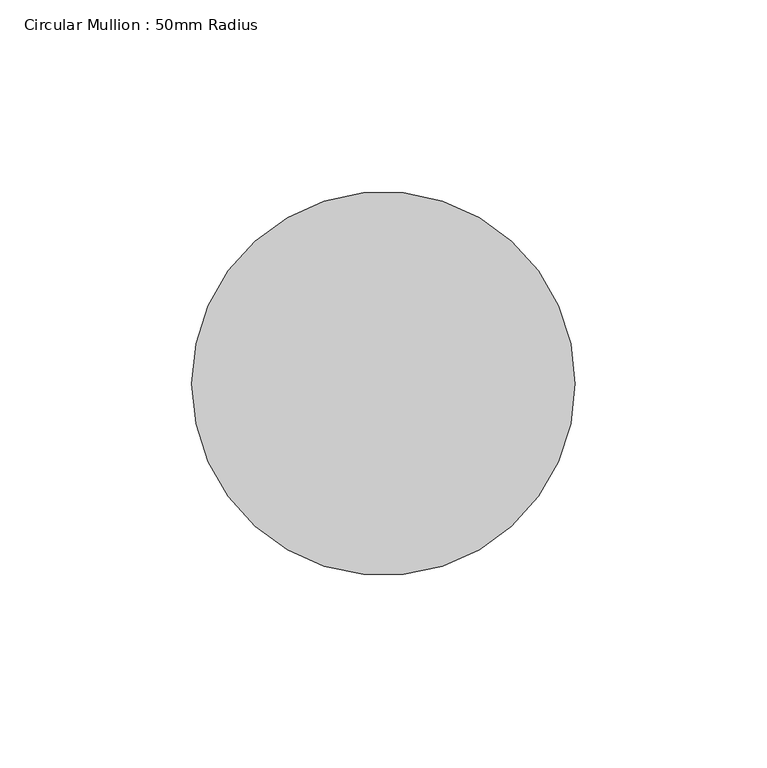
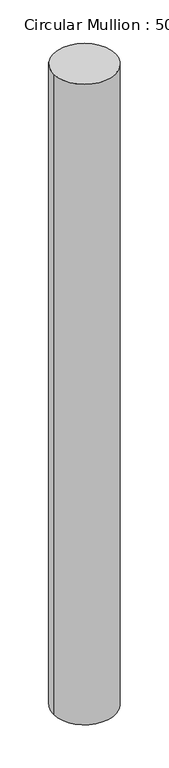
"""IFC4 building model written with IfcOpenShell, lengths in millimetres: member geometry, Circular Mullion : 50mm Radius."""

import ifcopenshell
import ifcopenshell.guid

model = None  # the IFC model being written
_history = None  # IfcOwnerHistory: only IFC2X3 demands one
_inside = {}  # id of a spatial element -> (the spatial element, [elements in it])
_under = {}  # id of a project, library or spatial element -> (it, [spatial elements below it])
_declared = {}  # id of a project -> (the project, [libraries it declares])
_typed = {}  # id of a type object -> (the type object, [elements of that type])
_made_of = {}  # id of a material, layer set ... -> (it, [elements and type objects made of it])


def new_model(schema):
    """Start an empty IFC model of exactly this schema.

    Asked for "IFC4X3", IfcOpenShell would pick the latest addendum, in which some entities
    have other attributes; the version numbers below select the first issue.
    IFC2X3 requires an IfcOwnerHistory on every rooted entity: one is made here for all.
    """
    global model, _history
    if schema == "IFC4X3":
        model = ifcopenshell.file(schema_version=(4, 3, 0, 0))
    else:
        model = ifcopenshell.file(schema=schema)
    _inside.clear()
    _under.clear()
    _declared.clear()
    _typed.clear()
    _made_of.clear()
    _history = None
    if model.schema == "IFC2X3":
        org = make("IfcOrganization", Name="unknown")
        user = make(
            "IfcPersonAndOrganization",
            ThePerson=make("IfcPerson", FamilyName="unknown"),
            TheOrganization=org,
        )
        app = make(
            "IfcApplication",
            ApplicationDeveloper=org,
            Version="unknown",
            ApplicationFullName="unknown",
            ApplicationIdentifier="unknown",
        )
        _history = make(
            "IfcOwnerHistory",
            OwningUser=user,
            OwningApplication=app,
            ChangeAction="ADDED",
            CreationDate=0,
        )
    return model


def make(cls, **values):
    """One entity of the class cls with the attributes given. An attribute that is None is left unset."""
    return model.create_entity(
        cls, **{name: value for name, value in values.items() if value is not None}
    )


def rooted(cls, **values):
    """An entity with a GlobalId (a new one), such as an element, a storey or a relation."""
    return make(cls, GlobalId=ifcopenshell.guid.new(), OwnerHistory=_history, **values)


def si_unit(unit_type, name, prefix=None):
    """IfcSIUnit, for example si_unit("LENGTHUNIT", "METRE", prefix="MILLI")."""
    return make("IfcSIUnit", UnitType=unit_type, Prefix=prefix, Name=name)


def assignment(units):
    """IfcUnitAssignment: the units of a project."""
    return None if units is None else make("IfcUnitAssignment", Units=units)


def point(xyz):
    """IfcCartesianPoint."""
    return None if xyz is None else make("IfcCartesianPoint", Coordinates=xyz)


def direction(xyz):
    """IfcDirection."""
    return None if xyz is None else make("IfcDirection", DirectionRatios=xyz)


def frame(location, z_axis=None, x_axis=None):
    """IfcAxis2Placement3D, a coordinate frame: its origin and axes. An axis left out is left unset."""
    return make(
        "IfcAxis2Placement3D",
        Location=point(location),
        Axis=direction(z_axis),
        RefDirection=direction(x_axis),
    )


def frame_2d(location, x_axis=None):
    """IfcAxis2Placement2D, a coordinate frame in the plane: its origin and x axis."""
    return make(
        "IfcAxis2Placement2D", Location=point(location), RefDirection=direction(x_axis)
    )


def origin():
    """The frame at (0, 0, 0) with its axes left unset."""
    return frame((0.0, 0.0, 0.0))


def origin_2d():
    """The frame at (0, 0) in the plane with its x axis left unset."""
    return frame_2d((0.0, 0.0))


def place(relative_to, where):
    """IfcLocalPlacement: puts the frame where relative to a parent placement (None: the world)."""
    return make(
        "IfcLocalPlacement", PlacementRelTo=relative_to, RelativePlacement=where
    )


def context(
    kind, dimensions, precision=None, world=None, true_north=None, identifier=None
):
    """IfcGeometricRepresentationContext, for example the 3D "Model" context."""
    return make(
        "IfcGeometricRepresentationContext",
        ContextIdentifier=identifier,
        ContextType=kind,
        CoordinateSpaceDimension=dimensions,
        Precision=precision,
        WorldCoordinateSystem=world,
        TrueNorth=true_north,
    )


def project(units=None, contexts=None):
    """IfcProject with its units and contexts."""
    return rooted(
        "IfcProject",
        Name="project",
        RepresentationContexts=contexts,
        UnitsInContext=assignment(units),
    )


def spatial(cls, under=None, at=None, **own):
    """A site, building, storey or space (cls), placed at a placement, below another one or the project."""
    s = rooted(cls, ObjectPlacement=at, **own)
    if under is not None:
        _under.setdefault(under.id(), (under, []))[1].append(s)
    return s


def circle_curve(where, radius):
    """IfcCircle in the frame where."""
    return make("IfcCircle", Position=where, Radius=radius)


def trimmed(basis, trim1, trim2, sense, master):
    """IfcTrimmedCurve: the piece of a basis curve between two trims."""
    return make(
        "IfcTrimmedCurve",
        BasisCurve=basis,
        Trim1=trim1,
        Trim2=trim2,
        SenseAgreement=sense,
        MasterRepresentation=master,
    )


def segment(curve, same_sense, transition):
    """IfcCompositeCurveSegment."""
    return make(
        "IfcCompositeCurveSegment",
        Transition=transition,
        SameSense=same_sense,
        ParentCurve=curve,
    )


def composite_curve(segments, self_intersect=None):
    """IfcCompositeCurve: segments joined end to end."""
    return make("IfcCompositeCurve", Segments=segments, SelfIntersect=self_intersect)


def outline(outer, holes=None, kind="AREA"):
    """IfcArbitraryClosedProfileDef: a profile drawn as a closed curve; with holes, ...WithVoids."""
    if holes is None:
        return make("IfcArbitraryClosedProfileDef", ProfileType=kind, OuterCurve=outer)
    return make(
        "IfcArbitraryProfileDefWithVoids",
        ProfileType=kind,
        OuterCurve=outer,
        InnerCurves=holes,
    )


def extrude(swept, where, along, depth):
    """IfcExtrudedAreaSolid: the profile swept, set in the frame where, extruded along a direction by depth."""
    return make(
        "IfcExtrudedAreaSolid",
        SweptArea=swept,
        Position=where,
        ExtrudedDirection=direction(along),
        Depth=depth,
    )


def shape(context_of_items, identifier, shape_type, items):
    """IfcShapeRepresentation: the items that make up one representation, for example the "Body"."""
    return make(
        "IfcShapeRepresentation",
        ContextOfItems=context_of_items,
        RepresentationIdentifier=identifier,
        RepresentationType=shape_type,
        Items=items,
    )


def source(mapping_origin, context_of_items, identifier, shape_type, items):
    """IfcRepresentationMap: a shape defined once, which mapped items show again and again."""
    return make(
        "IfcRepresentationMap",
        MappingOrigin=mapping_origin,
        MappedRepresentation=shape(context_of_items, identifier, shape_type, items),
    )


def transform(
    local_origin,
    x_axis=None,
    y_axis=None,
    z_axis=None,
    scale=None,
    scale2=None,
    scale3=None,
    uniform=True,
):
    """IfcCartesianTransformationOperator3D, or its non-uniform kind. x_axis, y_axis, z_axis: its Axis1, 2, 3."""
    if uniform:
        return make(
            "IfcCartesianTransformationOperator3D",
            Axis1=direction(x_axis),
            Axis2=direction(y_axis),
            LocalOrigin=point(local_origin),
            Scale=scale,
            Axis3=direction(z_axis),
        )
    return make(
        "IfcCartesianTransformationOperator3DnonUniform",
        Axis1=direction(x_axis),
        Axis2=direction(y_axis),
        LocalOrigin=point(local_origin),
        Scale=scale,
        Axis3=direction(z_axis),
        Scale2=scale2,
        Scale3=scale3,
    )


def mapped(mapping_source, mapping_target):
    """IfcMappedItem: shows the shape of a source again, moved by a transform."""
    return make(
        "IfcMappedItem", MappingSource=mapping_source, MappingTarget=mapping_target
    )


def made_of(thing, what):
    """Note that an element or type object is made of a material, layer set ...; save() writes the relation."""
    if what is not None:
        _made_of.setdefault(what.id(), (what, []))[1].append(thing)
    return thing


def element(
    cls,
    number,
    at=None,
    inside=None,
    cuts=None,
    type_object=None,
    material=None,
    context=None,
    identifier="Body",
    shape_type=None,
    held_by="IfcProductDefinitionShape",
    body=None,
    shapes=None,
    **own,
):
    """One element of the class cls, such as IfcWall. Its Tag is "e" and its number.

    at: its placement. inside: the storey or other place that contains it. cuts: it is an
    opening in that element (IfcRelVoidsElement). A single representation is given by context,
    identifier, shape_type and body (its items); several are given by shapes. held_by: the class
    of the entity that holds the representations. save() writes the other relations.
    """
    e = rooted(cls, Tag="e%d" % number, ObjectPlacement=at, **own)
    if body is not None:
        shapes = [shape(context, identifier, shape_type, body)]
    if shapes is not None:
        e.Representation = make(held_by, Representations=shapes)
    if inside is not None:
        _inside.setdefault(inside.id(), (inside, []))[1].append(e)
    if cuts is not None:
        rooted(
            "IfcRelVoidsElement", RelatingBuildingElement=cuts, RelatedOpeningElement=e
        )
    if type_object is not None:
        _typed.setdefault(type_object.id(), (type_object, []))[1].append(e)
    return made_of(e, material)


def aggregate(whole, parts):
    """IfcRelAggregates: a whole, such as a stair, and the parts it consists of."""
    return rooted("IfcRelAggregates", RelatingObject=whole, RelatedObjects=parts)


def save(model, path):
    """Write the relations noted so far, then the file.

    IfcRelAggregates (storeys below a building ...), IfcRelContainedInSpatialStructure (elements
    in a storey), IfcRelDefinesByType, IfcRelAssociatesMaterial and IfcRelDeclares: one each for
    every whole, place, type object, material and project.
    """
    for whole, parts in _under.values():
        aggregate(whole, parts)
    for where, things in _inside.values():
        rooted(
            "IfcRelContainedInSpatialStructure",
            RelatedElements=things,
            RelatingStructure=where,
        )
    for kind, things in _typed.values():
        rooted("IfcRelDefinesByType", RelatedObjects=things, RelatingType=kind)
    for what, things in _made_of.values():
        rooted("IfcRelAssociatesMaterial", RelatedObjects=things, RelatingMaterial=what)
    for by, libraries in _declared.values():
        rooted("IfcRelDeclares", RelatingContext=by, RelatedDefinitions=libraries)
    model.write(path)


def circular_mullion_50mm_radius_c50fe2aa(model_context):
    return source(origin(), model_context, "Body", "SweptSolid", [
        extrude(outline(composite_curve([segment(trimmed(circle_curve(origin_2d(), 50.0), [point((50.0, 0.0))], [point((-50.0, 0.0))], False, "CARTESIAN"), True, "CONTINUOUS"), segment(trimmed(circle_curve(origin_2d(), 50.0), [point((-50.0, 0.0))], [point((50.0, 0.0))], False, "CARTESIAN"), True, "CONTINUOUS")], self_intersect=False)), frame((0.0, 0.0, -1092.4865652), z_axis=(0.0, 0.0, 1.0), x_axis=(1.0, 0.0, 0.0)), (0.0, 0.0, 1.0), 1092.4865652),
    ])


if __name__ == "__main__":
    model = new_model("IFC4")
    model_context = context("Model", 3, world=origin())
    ifc_project = project(units=[si_unit("LENGTHUNIT", "METRE", prefix="MILLI")], contexts=[model_context])
    site = spatial("IfcSite", under=ifc_project)
    building = spatial("IfcBuilding", under=site)
    placement = place(None, origin())
    circular_mullion_50mm_radius_shape = circular_mullion_50mm_radius_c50fe2aa(model_context)
    element("IfcMember", 1, ObjectType="Circular Mullion : 50mm Radius", at=placement, inside=building, context=model_context, shape_type="MappedRepresentation", body=[
        mapped(circular_mullion_50mm_radius_shape, transform((0.0, 0.0, 0.0), x_axis=(1.0, 0.0, 0.0), y_axis=(0.0, 1.0, 0.0), z_axis=(0.0, 0.0, 1.0))),
    ])
    save(model, "model.ifc")

# Revit data of these elements
# Type "Circular Mullion : 50mm Radius"
#   built-in parameter 1007350 = 0.164042 (stored number, unit not read)
# Element 1 (IfcMember, "Circular Mullion : 50mm Radius")
#   Materials on its faces: "Aluminium"
# Materials
#   "Aluminium": class "Metal", colour RGB 247 247 247, transparency 0, Description = "Aluminium 6061", Cost = 0
